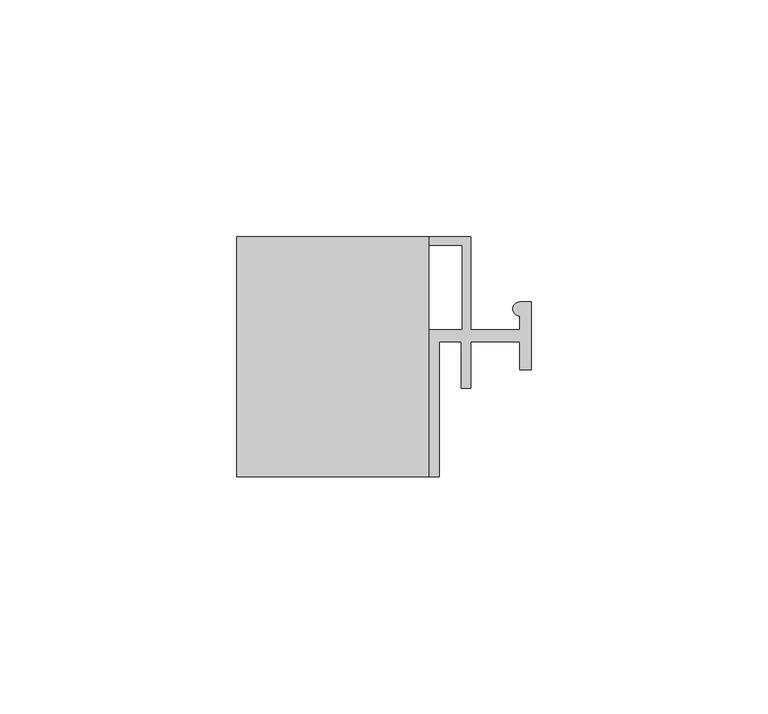
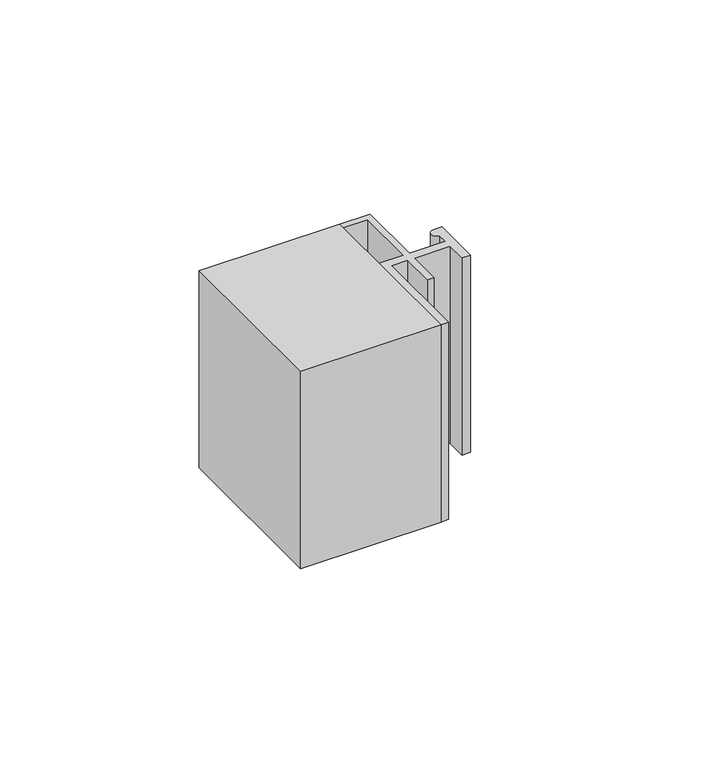
"""IFC4 building model written with IfcOpenShell, lengths in millimetres: proxy geometry, Generic Models 9:Generic Models 5:348123:Generic Models 5:348123 : Generic Models 9:Generic Models 5:348123:2 : Generic Models 9:Generic Models 5:348123:Generic Models 5:348123 : Generic Models 9:Generic Models 5:348123:301771."""

from ifc_helpers import new_model, si_unit, point, frame, frame_2d, origin, place, context, project, spatial, polyline, circle_curve, trimmed, segment, composite_curve, outline, extrude, source, transform, mapped, element, save


def generic_models_5576b47c(model_context):
    return source(origin(), model_context, "Body", "SweptSolid", [
        extrude(outline(polyline([(32083.0648622, 39220.6364592), (32083.0648622, 39271.4364592), (32123.6595224, 39271.4364592), (32123.6595224, 39220.6364592), (32083.0648622, 39220.6364592)])), frame((0.0, 0.0, 267346.9050805), z_axis=(0.0, 0.0, 1.0), x_axis=(1.0, 0.0, 0.0)), (0.0, 0.0, 1.0), 60.325),
        extrude(outline(composite_curve([segment(polyline([(32132.5371923, 39251.7083039), (32142.8944738, 39251.7083039), (32142.8944738, 39254.6675272)]), True, "CONTINUOUS"), segment(trimmed(circle_curve(frame_2d((32142.8944738, 39256.1471389)), 1.4796117), [point((32142.8944738, 39254.6675272))], [point((32142.8944738, 39257.6267505))], False, "CARTESIAN"), True, "CONTINUOUS"), segment(polyline([(32142.8944738, 39257.6267505), (32145.3604932, 39257.6267505), (32145.3604932, 39243.3238379), (32142.8944738, 39243.3238379), (32142.8944738, 39249.2422845), (32132.5371923, 39249.2422845), (32132.5371923, 39239.3782068), (32130.5643767, 39239.3782068), (32130.5643767, 39249.2422845), (32125.9282602, 39249.2422845), (32125.9282602, 39220.6364592), (32123.6595224, 39220.6364592), (32123.6595224, 39251.7083039), (32130.7616583, 39251.7083039), (32130.7616583, 39269.6609253), (32123.6595224, 39269.6609253), (32123.6595224, 39271.4364592), (32132.5371923, 39271.4364592), (32132.5371923, 39251.7083039)]), True, "CONTINUOUS")], self_intersect=False)), frame((0.0, 0.0, 267346.9050805), z_axis=(0.0, 0.0, 1.0), x_axis=(1.0, 0.0, 0.0)), (0.0, 0.0, 1.0), 60.325),
    ])


if __name__ == "__main__":
    model = new_model("IFC4")
    model_context = context("Model", 3, world=origin())
    ifc_project = project(units=[si_unit("LENGTHUNIT", "METRE", prefix="MILLI")], contexts=[model_context])
    site = spatial("IfcSite", under=ifc_project)
    building = spatial("IfcBuilding", under=site)
    placement = place(None, origin())
    generic_models_shape = generic_models_5576b47c(model_context)
    element("IfcBuildingElementProxy", 1, Name="Generic Models 9:Generic Models 5:348123:Generic Models 5:348123 : Generic Models 9:Generic Models 5:348123:2 : Generic Models 9:Generic Models 5:348123:Generic Models 5:348123 : Generic Models 9:Generic Models 5:348123:301771", ObjectType="Generic Models 9:Generic Models 5:348123:Generic Models 5:348123 : Generic Models 9:Generic Models 5:348123:2 : Generic Models 9:Generic Models 5:348123:Generic Models 5:348123 : Generic Models 9:Generic Models 5:348123:301771", at=placement, inside=building, context=model_context, shape_type="MappedRepresentation", body=[
        mapped(generic_models_shape, transform((0.0, 0.0, 0.0), x_axis=(1.0, 0.0, 0.0), y_axis=(0.0, 1.0, 0.0), z_axis=(0.0, 0.0, 1.0))),
    ])
    save(model, "model.ifc")

# Revit data of these elements
# Type "Generic Models 9:Generic Models 5:348123:Generic Models 5:348123 : Generic Models 9:Generic Models 5:348123:2 : Generic Models 9:Generic Models 5:348123:Generic Models 5:348123 : Generic Models 9:Generic Models 5:348123:301771"
#   NameOverride = "Generic Models 9:Generic Models 5:348123:Generic Models 5:348123 : Generic Models 9:Generic Models 5:348123:301771"
#   ObjectTypeOverride = "Generic Models 5:348123 : Generic Models 9:Generic Models 5:348123"
#   Reference = "Generic Models 5"
#   Tag = "301771"
# Element 1 (IfcBuildingElementProxy, "Generic Models 9:Generic Models 5:348123:Generic Models 5:348123 : Generic Models 9:Generic Models 5:348123:2 : Generic Models 9:Generic Models 5:348123:Generic Models 5:348123 : Generic Models 9:Generic Models 5:348123:301771")
#   Materials on its faces: "GA. STEEL CLIP AT EVERY SEAM IN POLYCARBONATE"
# Materials
#   "GA. STEEL CLIP AT EVERY SEAM IN POLYCARBONATE": class "Unassigned", colour RGB 120 120 120, transparency 0, Cost = 0
